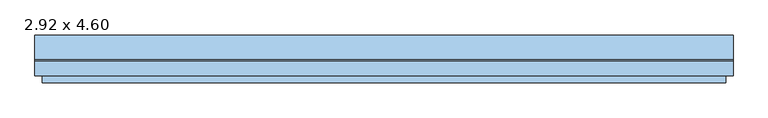
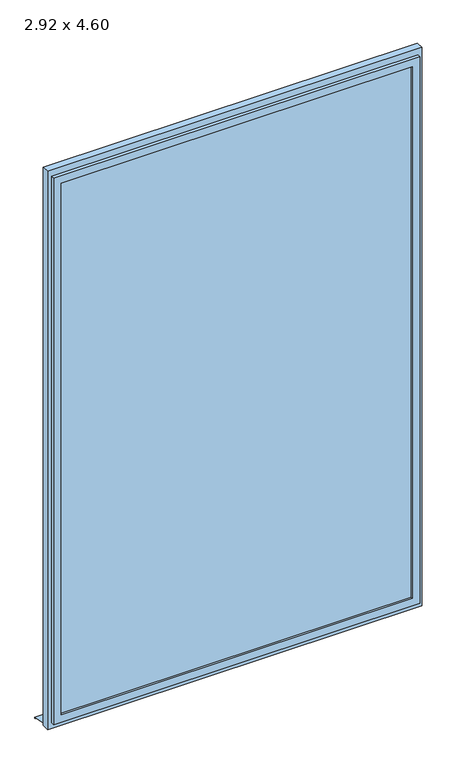
"""IFC4 building model written with IfcOpenShell, lengths in millimetres: window geometry, Fenstertür 1-flg : 2.92 x 4.60."""

from ifc_helpers import new_model, si_unit, frame, origin, place, context, project, spatial, polyline, outline, extrude, faceted_brep, source, transform, mapped, element, save


def window_2_92_x_4_60_476d09a5(model_context):
    return source(origin(), model_context, "Body", "SolidModel", [
        extrude(outline(polyline([(4600.0, 1460.0), (4600.0, -1460.0), (0.0, -1460.0), (0.0, 1460.0), (4600.0, 1460.0)]), holes=[polyline([(4520.0, 1400.0), (80.0, 1400.0), (80.0, -1400.0), (4520.0, -1400.0), (4520.0, 1400.0)])]), frame((0.0, -80.0, 0.0), z_axis=(0.0, 1.0, 0.0), x_axis=(0.0, 0.0, 1.0)), (0.0, 0.0, 1.0), 60.0),
        faceted_brep([(1430.0, -80.0, 4550.0), (1430.0, -110.0, 4550.0), (1430.0, -110.0, 50.0), (1430.0, -80.0, 50.0), (-1430.0, -110.0, 4550.0), (-1430.0, -110.0, 50.0), (1370.0, -110.0, 110.0), (-1370.0, -110.0, 110.0), (-1370.0, -110.0, 4490.0), (1370.0, -110.0, 4490.0), (-1430.0, -80.0, 50.0), (-1430.0, -80.0, 4550.0), (1400.0, -80.0, 4520.0), (-1400.0, -80.0, 4520.0), (-1400.0, -80.0, 80.0), (1400.0, -80.0, 80.0), (1400.0, -50.0, 4520.0), (1400.0, -50.0, 80.0), (-1400.0, -50.0, 80.0), (-1400.0, -50.0, 4520.0), (1370.0, -50.0, 4490.0), (-1370.0, -50.0, 4490.0), (-1370.0, -50.0, 110.0), (1370.0, -50.0, 110.0)], [[[0, 1, 2, 3]], [[1, 4, 5, 2], [6, 7, 8, 9]], [[3, 2, 5, 10]], [[3, 10, 11, 0], [12, 13, 14, 15]], [[16, 12, 15, 17]], [[17, 15, 14, 18]], [[17, 18, 19, 16], [20, 21, 22, 23]], [[9, 20, 23, 6]], [[6, 23, 22, 7]], [[10, 5, 4, 11]], [[18, 14, 13, 19]], [[7, 22, 21, 8]], [[11, 4, 1, 0]], [[19, 13, 12, 16]], [[8, 21, 20, 9]]]),
        extrude(outline(polyline([(-9.9778457, 20.0), (90.0, 0.0), (90.0, -10.0), (88.0, -10.0), (88.0, -1.6395366), (-10.1759277, 18.0), (-20.0, 18.0), (-20.0, 20.0), (-9.9778457, 20.0)])), frame((-1460.0, 0.0, 0.0), z_axis=(1.0, 0.0, 0.0), x_axis=(0.0, 1.0, 0.0)), (0.0, 0.0, 1.0), 2920.0),
        extrude(outline(polyline([(1370.0, -95.0), (-1370.0, -95.0), (-1370.0, -65.0), (1370.0, -65.0), (1370.0, -95.0)])), frame((0.0, 0.0, 110.0), z_axis=(0.0, 0.0, 1.0), x_axis=(1.0, 0.0, 0.0)), (0.0, 0.0, 1.0), 4380.0),
    ])


if __name__ == "__main__":
    model = new_model("IFC4")
    model_context = context("Model", 3, world=origin())
    ifc_project = project(units=[si_unit("LENGTHUNIT", "METRE", prefix="MILLI")], contexts=[model_context])
    site = spatial("IfcSite", under=ifc_project)
    building = spatial("IfcBuilding", under=site)
    placement = place(None, origin())
    window_2_92_x_4_60_shape = window_2_92_x_4_60_476d09a5(model_context)
    element("IfcWindow", 1, ObjectType="Fenstertür 1-flg : 2.92 x 4.60", at=placement, inside=building, context=model_context, shape_type="MappedRepresentation", body=[
        mapped(window_2_92_x_4_60_shape, transform((0.0, 0.0, 0.0), x_axis=(1.0, 0.0, 0.0), y_axis=(0.0, 1.0, 0.0), z_axis=(0.0, 0.0, 1.0))),
    ])
    save(model, "model.ifc")

# Revit data of these elements
# Type "Fenstertür 1-flg : 2.92 x 4.60"
#   Type Mark = "55"
#   Operation = "SinglePanel"
#   Construction Type Id = "SGL"
#   Keynote = "16.05.01"
#   Analytic Construction = "Große Fenster mit Einfachverglasung"
#   Visual Light Transmittance = 0.9
#   Solar Heat Gain Coefficient = 0.86
#   Rough Width = 2.920 m
#   Rough Height = 4.600 m
#   Heat Transfer Coefficient (U) = 5.5617 W/(m²·K)
#   Rahmentiefe = 0.060 m
#   Rahmenhöhe unten = 0.080 m
#   Höhe oberer  Rahmen = 0.080 m
#   Rahmenbreite = 0.060 m
#   Height = 4.600 m
#   Tiefe Flügel = 0.060 m
#   Flügelbreite = 0.060 m
#   Einbautiefe (von außen) [instance default] = 0.080 m
#   Width = 2.920 m
#   Sichtbarkeit Sturzlinien [instance default] = yes
#   Öffnungsrichtung oben [instance default] = yes
#   Öffnungsrichtung in Draufsicht anzeigen [instance default] = yes
#   Drehflügel 1 [instance default] = yes
#   Bild [instance default] = none
#   Glas [instance default] = none
#   Fensterflügel [instance default] = none
#   Äußere Fensterbank [instance default] = none
#   Wall Closure = (empty or 0)
# Element 1 (IfcWindow, "Fenstertür 1-flg : 2.92 x 4.60")
#   Materials on its faces: "Kunststoff - Weiß", "Glas"
# Materials
#   "Kunststoff - Weiß": class "Kunststoff", colour RGB 249 249 249, transparency 0, Cost = 0
#   "Glas": class "Glas", colour RGB 0 0 255, transparency 0.75, Comments = "Render-Darstellung nicht aktualisiert ", Cost = 0
